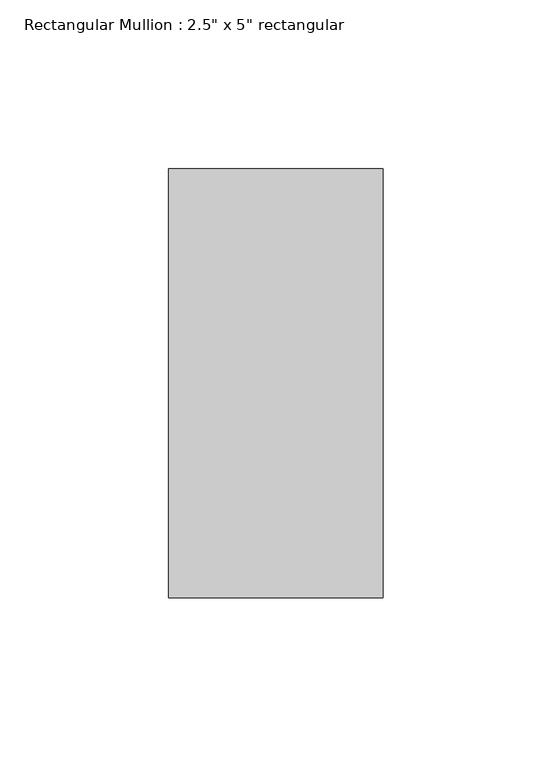
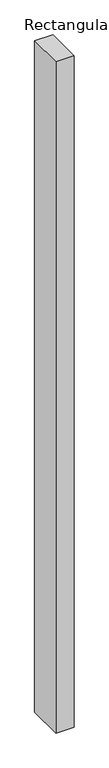
"""IFC4 building model written with IfcOpenShell, lengths in millimetres: member geometry."""

import ifcopenshell
import ifcopenshell.guid

model = None  # the IFC model being written
_history = None  # IfcOwnerHistory: only IFC2X3 demands one
_inside = {}  # id of a spatial element -> (the spatial element, [elements in it])
_under = {}  # id of a project, library or spatial element -> (it, [spatial elements below it])
_declared = {}  # id of a project -> (the project, [libraries it declares])
_typed = {}  # id of a type object -> (the type object, [elements of that type])
_made_of = {}  # id of a material, layer set ... -> (it, [elements and type objects made of it])


def new_model(schema):
    """Start an empty IFC model of exactly this schema.

    Asked for "IFC4X3", IfcOpenShell would pick the latest addendum, in which some entities
    have other attributes; the version numbers below select the first issue.
    IFC2X3 requires an IfcOwnerHistory on every rooted entity: one is made here for all.
    """
    global model, _history
    if schema == "IFC4X3":
        model = ifcopenshell.file(schema_version=(4, 3, 0, 0))
    else:
        model = ifcopenshell.file(schema=schema)
    _inside.clear()
    _under.clear()
    _declared.clear()
    _typed.clear()
    _made_of.clear()
    _history = None
    if model.schema == "IFC2X3":
        org = make("IfcOrganization", Name="unknown")
        user = make(
            "IfcPersonAndOrganization",
            ThePerson=make("IfcPerson", FamilyName="unknown"),
            TheOrganization=org,
        )
        app = make(
            "IfcApplication",
            ApplicationDeveloper=org,
            Version="unknown",
            ApplicationFullName="unknown",
            ApplicationIdentifier="unknown",
        )
        _history = make(
            "IfcOwnerHistory",
            OwningUser=user,
            OwningApplication=app,
            ChangeAction="ADDED",
            CreationDate=0,
        )
    return model


def make(cls, **values):
    """One entity of the class cls with the attributes given. An attribute that is None is left unset."""
    return model.create_entity(
        cls, **{name: value for name, value in values.items() if value is not None}
    )


def rooted(cls, **values):
    """An entity with a GlobalId (a new one), such as an element, a storey or a relation."""
    return make(cls, GlobalId=ifcopenshell.guid.new(), OwnerHistory=_history, **values)


def si_unit(unit_type, name, prefix=None):
    """IfcSIUnit, for example si_unit("LENGTHUNIT", "METRE", prefix="MILLI")."""
    return make("IfcSIUnit", UnitType=unit_type, Prefix=prefix, Name=name)


def assignment(units):
    """IfcUnitAssignment: the units of a project."""
    return None if units is None else make("IfcUnitAssignment", Units=units)


def point(xyz):
    """IfcCartesianPoint."""
    return None if xyz is None else make("IfcCartesianPoint", Coordinates=xyz)


def direction(xyz):
    """IfcDirection."""
    return None if xyz is None else make("IfcDirection", DirectionRatios=xyz)


def frame(location, z_axis=None, x_axis=None):
    """IfcAxis2Placement3D, a coordinate frame: its origin and axes. An axis left out is left unset."""
    return make(
        "IfcAxis2Placement3D",
        Location=point(location),
        Axis=direction(z_axis),
        RefDirection=direction(x_axis),
    )


def origin():
    """The frame at (0, 0, 0) with its axes left unset."""
    return frame((0.0, 0.0, 0.0))


def place(relative_to, where):
    """IfcLocalPlacement: puts the frame where relative to a parent placement (None: the world)."""
    return make(
        "IfcLocalPlacement", PlacementRelTo=relative_to, RelativePlacement=where
    )


def context(
    kind, dimensions, precision=None, world=None, true_north=None, identifier=None
):
    """IfcGeometricRepresentationContext, for example the 3D "Model" context."""
    return make(
        "IfcGeometricRepresentationContext",
        ContextIdentifier=identifier,
        ContextType=kind,
        CoordinateSpaceDimension=dimensions,
        Precision=precision,
        WorldCoordinateSystem=world,
        TrueNorth=true_north,
    )


def project(units=None, contexts=None):
    """IfcProject with its units and contexts."""
    return rooted(
        "IfcProject",
        Name="project",
        RepresentationContexts=contexts,
        UnitsInContext=assignment(units),
    )


def spatial(cls, under=None, at=None, **own):
    """A site, building, storey or space (cls), placed at a placement, below another one or the project."""
    s = rooted(cls, ObjectPlacement=at, **own)
    if under is not None:
        _under.setdefault(under.id(), (under, []))[1].append(s)
    return s


def polyline(points):
    """IfcPolyline through the points."""
    return make("IfcPolyline", Points=[point(p) for p in points])


def outline(outer, holes=None, kind="AREA"):
    """IfcArbitraryClosedProfileDef: a profile drawn as a closed curve; with holes, ...WithVoids."""
    if holes is None:
        return make("IfcArbitraryClosedProfileDef", ProfileType=kind, OuterCurve=outer)
    return make(
        "IfcArbitraryProfileDefWithVoids",
        ProfileType=kind,
        OuterCurve=outer,
        InnerCurves=holes,
    )


def extrude(swept, where, along, depth):
    """IfcExtrudedAreaSolid: the profile swept, set in the frame where, extruded along a direction by depth."""
    return make(
        "IfcExtrudedAreaSolid",
        SweptArea=swept,
        Position=where,
        ExtrudedDirection=direction(along),
        Depth=depth,
    )


def shape(context_of_items, identifier, shape_type, items):
    """IfcShapeRepresentation: the items that make up one representation, for example the "Body"."""
    return make(
        "IfcShapeRepresentation",
        ContextOfItems=context_of_items,
        RepresentationIdentifier=identifier,
        RepresentationType=shape_type,
        Items=items,
    )


def source(mapping_origin, context_of_items, identifier, shape_type, items):
    """IfcRepresentationMap: a shape defined once, which mapped items show again and again."""
    return make(
        "IfcRepresentationMap",
        MappingOrigin=mapping_origin,
        MappedRepresentation=shape(context_of_items, identifier, shape_type, items),
    )


def transform(
    local_origin,
    x_axis=None,
    y_axis=None,
    z_axis=None,
    scale=None,
    scale2=None,
    scale3=None,
    uniform=True,
):
    """IfcCartesianTransformationOperator3D, or its non-uniform kind. x_axis, y_axis, z_axis: its Axis1, 2, 3."""
    if uniform:
        return make(
            "IfcCartesianTransformationOperator3D",
            Axis1=direction(x_axis),
            Axis2=direction(y_axis),
            LocalOrigin=point(local_origin),
            Scale=scale,
            Axis3=direction(z_axis),
        )
    return make(
        "IfcCartesianTransformationOperator3DnonUniform",
        Axis1=direction(x_axis),
        Axis2=direction(y_axis),
        LocalOrigin=point(local_origin),
        Scale=scale,
        Axis3=direction(z_axis),
        Scale2=scale2,
        Scale3=scale3,
    )


def mapped(mapping_source, mapping_target):
    """IfcMappedItem: shows the shape of a source again, moved by a transform."""
    return make(
        "IfcMappedItem", MappingSource=mapping_source, MappingTarget=mapping_target
    )


def made_of(thing, what):
    """Note that an element or type object is made of a material, layer set ...; save() writes the relation."""
    if what is not None:
        _made_of.setdefault(what.id(), (what, []))[1].append(thing)
    return thing


def element(
    cls,
    number,
    at=None,
    inside=None,
    cuts=None,
    type_object=None,
    material=None,
    context=None,
    identifier="Body",
    shape_type=None,
    held_by="IfcProductDefinitionShape",
    body=None,
    shapes=None,
    **own,
):
    """One element of the class cls, such as IfcWall. Its Tag is "e" and its number.

    at: its placement. inside: the storey or other place that contains it. cuts: it is an
    opening in that element (IfcRelVoidsElement). A single representation is given by context,
    identifier, shape_type and body (its items); several are given by shapes. held_by: the class
    of the entity that holds the representations. save() writes the other relations.
    """
    e = rooted(cls, Tag="e%d" % number, ObjectPlacement=at, **own)
    if body is not None:
        shapes = [shape(context, identifier, shape_type, body)]
    if shapes is not None:
        e.Representation = make(held_by, Representations=shapes)
    if inside is not None:
        _inside.setdefault(inside.id(), (inside, []))[1].append(e)
    if cuts is not None:
        rooted(
            "IfcRelVoidsElement", RelatingBuildingElement=cuts, RelatedOpeningElement=e
        )
    if type_object is not None:
        _typed.setdefault(type_object.id(), (type_object, []))[1].append(e)
    return made_of(e, material)


def aggregate(whole, parts):
    """IfcRelAggregates: a whole, such as a stair, and the parts it consists of."""
    return rooted("IfcRelAggregates", RelatingObject=whole, RelatedObjects=parts)


def save(model, path):
    """Write the relations noted so far, then the file.

    IfcRelAggregates (storeys below a building ...), IfcRelContainedInSpatialStructure (elements
    in a storey), IfcRelDefinesByType, IfcRelAssociatesMaterial and IfcRelDeclares: one each for
    every whole, place, type object, material and project.
    """
    for whole, parts in _under.values():
        aggregate(whole, parts)
    for where, things in _inside.values():
        rooted(
            "IfcRelContainedInSpatialStructure",
            RelatedElements=things,
            RelatingStructure=where,
        )
    for kind, things in _typed.values():
        rooted("IfcRelDefinesByType", RelatedObjects=things, RelatingType=kind)
    for what, things in _made_of.values():
        rooted("IfcRelAssociatesMaterial", RelatedObjects=things, RelatingMaterial=what)
    for by, libraries in _declared.values():
        rooted("IfcRelDeclares", RelatingContext=by, RelatedDefinitions=libraries)
    model.write(path)


def member_da42f391(model_context):
    return source(origin(), model_context, "Body", "SweptSolid", [
        extrude(outline(polyline([(31.75, 63.5), (31.75, -63.5), (-31.75, -63.5), (-31.75, 63.5), (31.75, 63.5)])), frame((0.0, 0.0, -2461.8630718), z_axis=(0.0, 0.0, 1.0), x_axis=(1.0, 0.0, 0.0)), (0.0, 0.0, 1.0), 2461.8630718),
    ])


if __name__ == "__main__":
    model = new_model("IFC4")
    model_context = context("Model", 3, world=origin())
    ifc_project = project(units=[si_unit("LENGTHUNIT", "METRE", prefix="MILLI")], contexts=[model_context])
    site = spatial("IfcSite", under=ifc_project)
    building = spatial("IfcBuilding", under=site)
    placement = place(None, origin())
    member_shape = member_da42f391(model_context)
    element("IfcMember", 1, ObjectType="Rectangular Mullion : 2.5\" x 5\" rectangular", at=placement, inside=building, context=model_context, shape_type="MappedRepresentation", body=[
        mapped(member_shape, transform((0.0, 0.0, 0.0), x_axis=(1.0, 0.0, 0.0), y_axis=(0.0, 1.0, 0.0), z_axis=(0.0, 0.0, 1.0))),
    ])
    save(model, "model.ifc")

# Revit data of these elements
# Type "Rectangular Mullion : 2.5\" x 5\" rectangular"
#   built-in parameter 1007304 = 0.416667 (stored number, unit not read)
#   built-in parameter 1007301 = 0.104167 (stored number, unit not read)
#   built-in parameter 1007300 = 0.104167 (stored number, unit not read)
# Element 1 (IfcMember, "Rectangular Mullion : 2.5\" x 5\" rectangular")
#   Materials on its faces: "Aluminum"
# Materials
#   "Aluminum": class "Metal", colour RGB 247 247 247, transparency 0, Description = "Aluminum 6061", Cost = 0
